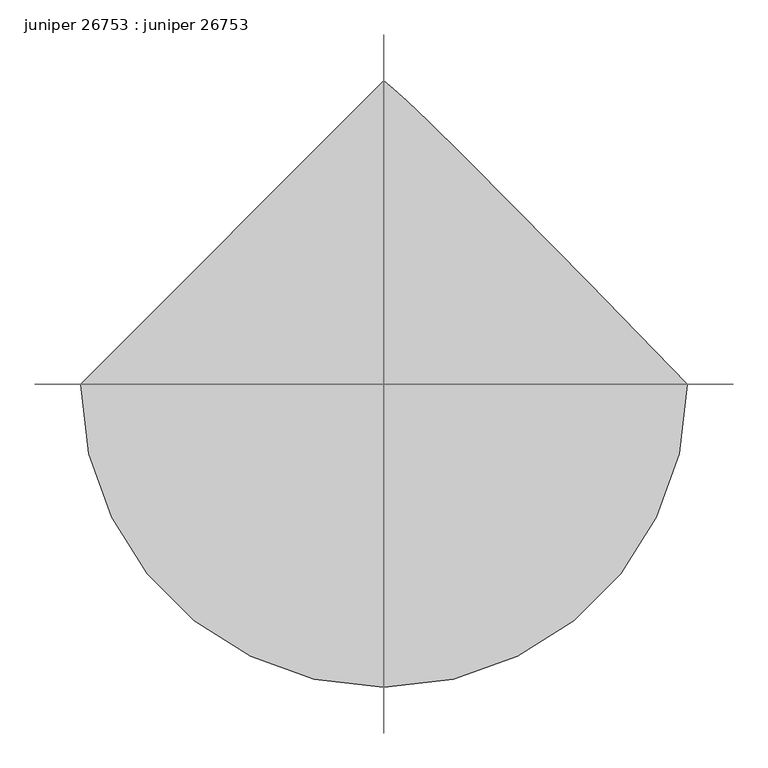
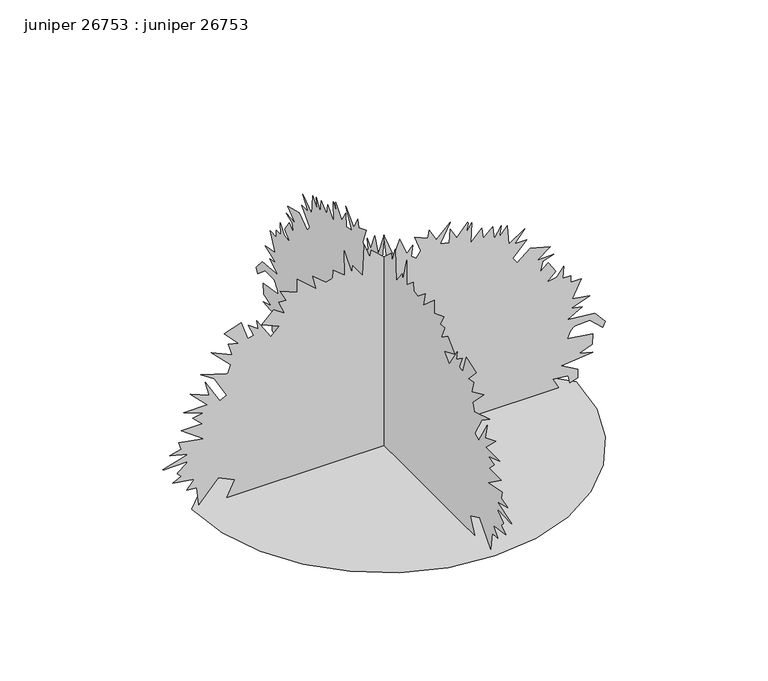
"""IFC4 building model written with IfcOpenShell, lengths in millimetres: proxy geometry, juniper 26753 : juniper 26753."""

from ifc_helpers import new_model, si_unit, origin, place, context, project, spatial, triangles, source, transform, mapped, element, save


def juniper_26753_juniper_26753_31b723d7(model_context):
    return source(origin(), model_context, "Body", "Tessellation", [
        triangles([(-789.9406637, 0.0, 7.34e-05), (-769.0593075, -181.0023239, 7.34e-05), (-709.58256, -347.2233553, 7.34e-05), (-616.27561, -493.9033919, 7.34e-05), (-493.9033919, -616.27561, 7.34e-05), (-347.2233553, -709.58256, 7.34e-05), (-181.0023239, -769.0593075, 7.34e-05), (3.45e-05, -789.9406637, 7.34e-05), (181.0025783, -769.0593075, 7.34e-05), (347.2233553, -709.58256, 7.34e-05), (493.9033919, -616.27561, 7.34e-05), (616.27561, -493.9033919, 7.34e-05), (709.58256, -347.2233553, 7.34e-05), (769.0593075, -181.0023239, 7.34e-05), (789.9406637, 6.91e-05, 7.34e-05), (533.2276995, 263.324552, 7.34e-05), (342.9129716, 457.2003633, 7.34e-05), (207.9314215, 593.1996929, 7.34e-05), (117.2157559, 682.8973429, 7.34e-05), (59.6994447, 737.8705862, 7.34e-05), (24.316455, 769.6942978, 7.34e-05), (-0.0001036, 789.9406637, 7.34e-05), (-3.6e-06, -645.975832, 2.9e-06), (1e-06, -614.2334381, 66.8205943), (0.0, -680.8932501, 98.5983058), (0.0, -760.2505428, 9.7171587), (0.0, -769.7755428, 85.9010885), (0.0, -811.0403933, 89.0753315), (0.0, -779.2979994, 127.1672379), (0.0, -868.1777487, 139.8647005), (0.0, -833.2603306, 158.9106491), (0.0, -849.1328356, 174.7823729), (2e-07, -847.0271502, 178.352086), (-1e-07, -810.1082554, 207.9471727), (0.0, -807.8654417, 212.8742702), (2e-07, -903.2958086, 210.5745559), (0.0, -909.4452152, 212.8742702), (0.0, -804.6929609, 244.6174271), (0.0, -880.8752295, 263.6623765), (0.0, -833.2603306, 276.3598392), (0.0, -842.7828598, 308.1047765), (0.0, -741.2056297, 289.0573199), (0.0, -833.2603306, 355.7196754), (0.0, -747.5530621, 355.7196754), (0.0, -785.6455044, 393.8120813), (0.0, -741.2056297, 403.3345379), (0.0, -823.737874, 431.9019439), (0.0, -725.3331247, 431.9019439), (0.0, -795.1679609, 501.7392872), (0.0, -718.9856924, 469.9943499), (0.0, -734.8581247, 533.4817174), (0.0, -674.5432743, 431.9019439), (0.0, -645.975832, 444.5994246), (0.0, -696.7657551, 533.4817174), (0.0, -753.9031105, 571.5741234), (0.0, -642.8008804, 536.6567053), (0.0, -630.1033997, 571.5741234), (0.0, -709.4632359, 650.9314161), (0.0, -623.7558947, 612.8389738), (0.0, -639.6283997, 663.6288969), (0.0, -598.3609694, 654.1063677), (0.0, -655.4982885, 714.4187473), (0.0, -585.663525, 739.8137089), (0.0, -560.2685635, 660.4538727), (0.0, -534.8736382, 666.8038485), (0.0, -557.0935756, 717.5912281), (0.0, -515.8286888, 689.0237858), (6e-07, -522.1761575, 724.2739597), (0.0, -465.0388021, 635.0589111), (0.0, -430.1214203, 669.9763292), (0.0, -503.131208, 701.7212666), (0.0, -452.3413576, 749.3361654), (0.0, -407.901483, 717.5912281), (0.0, -433.2964082, 774.731127), (0.0, -401.5514709, 771.5561028), (0.0, -426.9463961, 819.1710016), (0.0, -357.1115962, 790.6010159), (0.0, -357.1115962, 847.7409147), (0.0, -277.7543035, 777.9035351), (0.0, -293.6242287, 838.2159147), (0.0, -239.6616431, 793.7760401), (0.0, -211.0929654, 800.1260159), (0.0, -207.9182137, 835.043434), (0.0, -160.303333, 796.9510643), (0.0, -163.4780847, 904.8782701), (0.0, -131.7346644, 796.9510643), (0.0, -128.560167, 825.518434), (0.0, -87.2937723, 768.3810785), (0.0, -80.9452954, 901.7032459), (0.0, -58.7248448, 838.2159147), (0.0, -52.3763679, 866.7858278), (0.0, 11.1100709, 809.6484724), (0.0, -1.5869882, 914.4007267), (0.0, 39.6794049, 809.6484724), (0.0, 65.073835, 873.1333328), (0.0, 93.6427671, 800.1260159), (0.0, 119.037447, 828.6934582), (0.0, 112.6887157, 784.2535835), (0.0, 131.7349187, 768.3810785), (0.0, 150.7808674, 793.7760401), (0.0, 125.3861874, 860.4383955), (0.0, 179.3497903, 838.2159147), (0.0, 185.698022, 869.9608521), (0.0, 214.2674628, 819.1710016), (0.0, 271.4042913, 876.308357), (0.0, 230.1389141, 796.9510643), (0.0, 268.2318287, 787.4285351), (0.0, 271.4042913, 844.5658905), (0.0, 299.9742408, 796.9510643), (0.0, 342.3973417, 848.8686802), (0.0, 344.7290671, 848.6756687), (0.0, 345.397086, 844.7309967), (0.0, 338.0666468, 806.4735209), (0.0, 360.2865841, 841.3909389), (0.0, 357.1115962, 755.6835978), (0.0, 401.5540143, 803.2984966), (0.0, 407.901483, 758.858622), (0.0, 445.993889, 793.7760401), (0.0, 452.3413576, 739.8137089), (0.0, 480.9112707, 787.4285351), (0.0, 474.5612949, 739.8137089), (0.0, 506.3062323, 777.9035351), (0.0, 512.6537009, 695.3712908), (0.0, 579.3160563, 739.8137089), (0.0, 538.0486261, 689.0237858), (0.0, 585.663525, 689.0237858), (0.0, 528.5261696, 628.7114788), (0.0, 547.5710827, 603.3165173), (0.0, 601.5359937, 647.7563919), (0.0, 684.0682743, 625.5364546), (0.0, 630.1033997, 584.2716042), (0.0, 696.7657551, 587.4440486), (0.0, 652.3258804, 571.5741234), (0.0, 642.8008804, 530.3066932), (0.0, 674.5458178, 558.8766426), (0.0, 706.2882116, 511.2617801), (0.0, 668.1957693, 476.344362), (0.0, 709.4632359, 482.6918306), (0.0, 738.0306055, 520.7842366), (0.0, 734.8581247, 469.9943499), (0.0, 766.6005186, 469.9943499), (0.0, 766.6005186, 441.4269439), (0.0, 811.0403933, 441.4269439), (0.0, 772.9480236, 368.4171198), (0.0, 845.9578114, 355.7196754), (0.0, 769.7755428, 327.1497259), (0.0, 814.2154175, 317.6272694), (0.0, 753.9031105, 282.7098513), (0.0, 865.0053406, 273.1873765), (0.0, 909.4452152, 222.3972354), (0.0, 899.922686, 200.1767894), (0.0, 845.9578114, 247.7916701), (0.0, 785.3051182, 246.4035645), (0.0, 777.2710882, 242.5165924), (0.0, 770.76618, 236.5473347), (0.0, 765.4803835, 228.9123538), (0.0, 761.1116095, 220.0279215), (0.0, 757.3549347, 210.3106367), (0.0, 753.9031105, 200.1767894), (0.0, 858.6552921, 184.3053381), (0.0, 855.4828114, 139.8647005), (0.0, 801.5179367, 120.8187518), (0.0, 858.6552921, 104.9470462), (0.0, 728.508149, 92.2498288), (0.0, 795.1705044, 54.1576681), (0.0, 795.1705044, 16.0658174), (0.0, 763.4255671, 6.5428419), (0.0, 757.0780621, 38.2862123), (0.0, 693.5907309, 44.6346938), (0.0, 718.9856924, 0.1941814), (-645.975832, 0.000119, 0.0), (-614.2334381, 0.0001104, 66.8205943), (-680.8932501, 0.0001095, 98.5983058), (-760.2505428, 0.0001148, 9.7171587), (-769.7755428, 0.0001102, 85.9010885), (-811.0403933, 0.0001101, 89.0753315), (-779.2979994, 0.0001078, 127.1672379), (-868.1777487, 0.000107, 139.8647005), (-833.2603306, 0.0001059, 158.9106491), (-849.1328356, 0.0001049, 174.7823729), (-847.0271502, 0.0001045, 178.352086), (-810.1082554, 0.000103, 207.9471727), (-807.8654417, 0.0001027, 212.8742702), (-903.2958086, 0.0001026, 210.5745559), (-909.4452152, 0.0001027, 212.8742702), (-804.6929609, 0.0001008, 244.6174271), (-880.8752295, 9.97e-05, 263.6623765), (-833.2603306, 9.89e-05, 276.3598392), (-842.7828598, 9.7e-05, 308.1047765), (-741.2056297, 9.81e-05, 289.0573199), (-833.2603306, 9.42e-05, 355.7196754), (-747.5530621, 9.42e-05, 355.7196754), (-785.6455044, 9.19e-05, 393.8120813), (-741.2056297, 9.13e-05, 403.3345379), (-823.737874, 8.96e-05, 431.9019439), (-725.3331247, 8.96e-05, 431.9019439), (-795.1679609, 8.55e-05, 501.7367437), (-718.9856924, 8.74e-05, 469.9943499), (-734.8581247, 8.36e-05, 533.4817174), (-674.5458178, 8.96e-05, 431.9019439), (-645.975832, 8.89e-05, 444.5994246), (-696.7657551, 8.36e-05, 533.4817174), (-753.9031105, 8.13e-05, 571.5741234), (-642.8008804, 8.34e-05, 536.6567053), (-630.1033997, 8.13e-05, 571.5741234), (-709.4632359, 7.66e-05, 650.9314161), (-623.7558947, 7.88e-05, 612.8389738), (-639.6283997, 7.58e-05, 663.6288969), (-598.3609694, 7.64e-05, 654.1063677), (-655.4982885, 7.28e-05, 714.4187473), (-585.663525, 7.13e-05, 739.8137089), (-560.2685635, 7.6e-05, 660.4538727), (-534.8736382, 7.56e-05, 666.8038485), (-557.0935756, 7.26e-05, 717.5912281), (-515.8286888, 7.43e-05, 689.0237858), (-522.1761575, 7.16e-05, 724.2739597), (-465.0388021, 7.75e-05, 635.0589111), (-430.1214203, 7.54e-05, 669.9763292), (-503.131208, 7.35e-05, 701.7212666), (-452.3413576, 7.07e-05, 749.3361654), (-407.901483, 7.26e-05, 717.5912281), (-433.2964082, 6.92e-05, 774.731127), (-401.5540143, 6.94e-05, 771.5561028), (-426.9463961, 6.65e-05, 819.1710016), (-357.1115962, 6.82e-05, 790.6010159), (-357.1115962, 6.48e-05, 847.7409147), (-277.7543035, 6.9e-05, 777.9035351), (-293.6242287, 6.54e-05, 838.2159147), (-239.6616431, 6.81e-05, 793.7760401), (-211.0929654, 6.77e-05, 800.1260159), (-207.918468, 6.56e-05, 835.043434), (-160.303333, 6.79e-05, 796.9510643), (-163.4780847, 6.14e-05, 904.8782701), (-131.7349187, 6.79e-05, 796.9510643), (-128.560167, 6.62e-05, 825.518434), (-87.2940267, 6.96e-05, 768.3810785), (-80.9452954, 6.16e-05, 901.7032459), (-58.7250992, 6.54e-05, 838.2159147), (-52.3766177, 6.37e-05, 866.7858278), (11.1099687, 6.71e-05, 809.6484724), (-1.5870796, 6.09e-05, 914.4007267), (39.6791505, 6.71e-05, 809.6484724), (65.073835, 6.33e-05, 873.1333328), (93.6427671, 6.77e-05, 800.1260159), (119.037447, 6.6e-05, 828.6934582), (112.6887157, 6.86e-05, 784.2535835), (131.7346644, 6.96e-05, 768.3810785), (150.780613, 6.81e-05, 793.7760401), (125.3861874, 6.41e-05, 860.4358521), (179.349536, 6.54e-05, 838.2159147), (185.698022, 6.35e-05, 869.9608521), (214.2672084, 6.65e-05, 819.1710016), (271.4042913, 6.31e-05, 876.308357), (230.1389141, 6.79e-05, 796.9510643), (268.2318287, 6.84e-05, 787.4285351), (271.4042913, 6.5e-05, 844.5658905), (299.9742408, 6.79e-05, 796.9510643), (342.3973417, 6.48e-05, 848.8686802), (344.7290671, 6.48e-05, 848.6756687), (345.3945425, 6.5e-05, 844.7309967), (338.0666468, 6.73e-05, 806.4735209), (360.2865841, 6.52e-05, 841.3909389), (357.1115962, 7.03e-05, 755.6835978), (401.5514709, 6.75e-05, 803.2984966), (407.901483, 7.01e-05, 758.858622), (445.993889, 6.81e-05, 793.7760401), (452.3413576, 7.13e-05, 739.8137089), (480.9112707, 6.84e-05, 787.4285351), (474.5612949, 7.13e-05, 739.8137089), (506.3062323, 6.9e-05, 777.9035351), (512.6537009, 7.39e-05, 695.3712908), (579.3160563, 7.13e-05, 739.8137089), (538.0486261, 7.43e-05, 689.0237858), (585.663525, 7.43e-05, 689.0237858), (528.5261696, 7.79e-05, 628.7114788), (547.5710827, 7.94e-05, 603.3165173), (601.5359937, 7.68e-05, 647.7563919), (684.0682743, 7.81e-05, 625.5364546), (630.1033997, 8.05e-05, 584.2716042), (696.7657551, 8.04e-05, 587.4440486), (652.3258804, 8.13e-05, 571.5741234), (642.8008804, 8.38e-05, 530.3066932), (674.5458178, 8.21e-05, 558.8766426), (706.2882116, 8.49e-05, 511.2617801), (668.1957693, 8.7e-05, 476.344362), (709.4632359, 8.66e-05, 482.6918306), (738.0306055, 8.43e-05, 520.7842366), (734.8581247, 8.74e-05, 469.9943499), (766.6005186, 8.74e-05, 469.9943499), (766.6005186, 8.91e-05, 441.4269439), (811.0403933, 8.91e-05, 441.4269439), (772.9480236, 9.34e-05, 368.4171198), (845.9578114, 9.42e-05, 355.7196754), (769.7755428, 9.59e-05, 327.1497259), (814.2154175, 9.64e-05, 317.6272694), (753.9031105, 9.85e-05, 282.7098513), (865.0053406, 9.91e-05, 273.1873765), (909.4452152, 0.0001021, 222.3972354), (899.922686, 0.0001034, 200.1767894), (845.9578114, 0.0001006, 247.7916701), (785.3051182, 0.0001007, 246.4035645), (777.2710882, 0.0001009, 242.5165924), (770.76618, 0.0001013, 236.5473347), (765.4803835, 0.0001017, 228.9123538), (761.1116095, 0.0001023, 220.0279215), (757.3549347, 0.0001028, 210.3106367), (753.9031105, 0.0001034, 200.1767894), (858.6552921, 0.0001044, 184.3050838), (855.4828114, 0.000107, 139.8647005), (801.5179367, 0.0001082, 120.8187518), (858.6552921, 0.0001091, 104.9470462), (728.508149, 0.0001099, 92.2495745), (795.1705044, 0.0001121, 54.1576681), (795.1705044, 0.0001144, 16.0658174), (763.4255671, 0.000115, 6.5428419), (757.0780621, 0.0001131, 38.2862123), (693.5907309, 0.0001127, 44.6346938), (718.9856924, 0.0001154, 0.1941786)], [[21, 22, 1], [20, 21, 1], [19, 20, 1], [18, 19, 1], [17, 18, 1], [17, 1, 2], [17, 2, 3], [17, 3, 4], [16, 17, 4], [16, 4, 5], [16, 5, 6], [16, 6, 7], [16, 7, 8], [16, 8, 9], [16, 9, 10], [16, 10, 11], [16, 11, 12], [15, 16, 12], [14, 15, 12], [13, 14, 12], [92, 93, 94], [84, 85, 86], [54, 55, 56], [50, 51, 52], [131, 132, 133], [123, 124, 125], [104, 105, 106], [46, 47, 48], [57, 58, 59], [88, 89, 90], [48, 49, 50], [67, 68, 69], [119, 120, 121], [162, 163, 164], [38, 39, 40], [113, 114, 115], [144, 145, 146], [65, 66, 67], [138, 139, 140], [96, 97, 98], [107, 108, 109], [79, 80, 81], [42, 43, 44], [29, 30, 31], [36, 37, 38], [75, 76, 77], [102, 103, 104], [146, 147, 148], [86, 87, 88], [94, 95, 96], [121, 122, 123], [125, 126, 127], [100, 101, 102], [77, 78, 79], [25, 26, 27], [115, 116, 117], [129, 130, 131], [117, 118, 119], [27, 28, 29], [82, 83, 84], [44, 45, 46], [48, 50, 52], [59, 60, 61], [169, 170, 23], [73, 74, 75], [90, 91, 92], [142, 143, 144], [40, 41, 42], [38, 40, 42], [169, 23, 24], [53, 54, 56], [61, 62, 63], [61, 63, 64], [70, 71, 72], [70, 72, 73], [150, 151, 152], [149, 150, 152], [148, 149, 152], [148, 152, 153], [128, 129, 131], [148, 153, 154], [35, 36, 38], [134, 135, 136], [134, 136, 137], [65, 67, 69], [166, 167, 168], [165, 166, 168], [164, 165, 168], [164, 168, 169], [88, 90, 92], [140, 141, 142], [100, 102, 104], [159, 160, 161], [159, 161, 162], [25, 27, 29], [123, 125, 127], [148, 154, 155], [100, 104, 106], [110, 111, 112], [109, 110, 112], [109, 112, 113], [109, 113, 115], [31, 32, 33], [131, 133, 134], [159, 162, 164], [128, 131, 134], [46, 48, 52], [73, 75, 77], [73, 77, 79], [29, 31, 33], [29, 33, 34], [44, 46, 52], [148, 155, 156], [164, 169, 24], [159, 164, 24], [158, 159, 24], [157, 158, 24], [156, 157, 24], [148, 156, 24], [146, 148, 24], [144, 146, 24], [142, 144, 24], [140, 142, 24], [138, 140, 24], [137, 138, 24], [134, 137, 24], [128, 134, 24], [127, 128, 24], [123, 127, 24], [121, 123, 24], [119, 121, 24], [117, 119, 24], [115, 117, 24], [109, 115, 24], [107, 109, 24], [106, 107, 24], [106, 24, 25], [106, 25, 29], [106, 29, 34], [106, 34, 35], [106, 35, 38], [106, 38, 42], [106, 42, 44], [106, 44, 52], [106, 52, 53], [106, 53, 56], [99, 100, 106], [99, 106, 56], [99, 56, 57], [98, 99, 57], [96, 98, 57], [94, 96, 57], [59, 61, 64], [57, 59, 64], [70, 73, 79], [64, 65, 69], [57, 64, 69], [94, 57, 69], [84, 86, 88], [88, 92, 94], [88, 94, 69], [88, 69, 70], [88, 70, 79], [84, 88, 79], [82, 84, 79], [82, 79, 81], [240, 241, 242], [232, 233, 234], [202, 203, 204], [198, 199, 200], [279, 280, 281], [271, 272, 273], [252, 253, 254], [194, 195, 196], [205, 206, 207], [236, 237, 238], [196, 197, 198], [215, 216, 217], [267, 268, 269], [310, 311, 312], [186, 187, 188], [261, 262, 263], [292, 293, 294], [213, 214, 215], [286, 287, 288], [244, 245, 246], [255, 256, 257], [227, 228, 229], [190, 191, 192], [177, 178, 179], [184, 185, 186], [223, 224, 225], [250, 251, 252], [294, 295, 296], [234, 235, 236], [242, 243, 244], [269, 270, 271], [273, 274, 275], [248, 249, 250], [225, 226, 227], [173, 174, 175], [263, 264, 265], [277, 278, 279], [265, 266, 267], [175, 176, 177], [230, 231, 232], [192, 193, 194], [196, 198, 200], [207, 208, 209], [317, 318, 171], [221, 222, 223], [238, 239, 240], [290, 291, 292], [188, 189, 190], [186, 188, 190], [317, 171, 172], [201, 202, 204], [209, 210, 211], [209, 211, 212], [218, 219, 220], [218, 220, 221], [298, 299, 300], [297, 298, 300], [296, 297, 300], [296, 300, 301], [276, 277, 279], [296, 301, 302], [183, 184, 186], [282, 283, 284], [282, 284, 285], [213, 215, 217], [314, 315, 316], [313, 314, 316], [312, 313, 316], [312, 316, 317], [236, 238, 240], [288, 289, 290], [248, 250, 252], [307, 308, 309], [307, 309, 310], [173, 175, 177], [271, 273, 275], [296, 302, 303], [248, 252, 254], [258, 259, 260], [257, 258, 260], [257, 260, 261], [257, 261, 263], [179, 180, 181], [279, 281, 282], [307, 310, 312], [276, 279, 282], [194, 196, 200], [221, 223, 225], [221, 225, 227], [177, 179, 181], [177, 181, 182], [192, 194, 200], [296, 303, 304], [312, 317, 172], [307, 312, 172], [306, 307, 172], [305, 306, 172], [304, 305, 172], [296, 304, 172], [294, 296, 172], [292, 294, 172], [290, 292, 172], [288, 290, 172], [286, 288, 172], [285, 286, 172], [282, 285, 172], [276, 282, 172], [275, 276, 172], [271, 275, 172], [269, 271, 172], [267, 269, 172], [265, 267, 172], [263, 265, 172], [257, 263, 172], [255, 257, 172], [254, 255, 172], [254, 172, 173], [254, 173, 177], [254, 177, 182], [254, 182, 183], [254, 183, 186], [254, 186, 190], [254, 190, 192], [254, 192, 200], [254, 200, 201], [254, 201, 204], [247, 248, 254], [247, 254, 204], [247, 204, 205], [246, 247, 205], [244, 246, 205], [242, 244, 205], [207, 209, 212], [205, 207, 212], [218, 221, 227], [212, 213, 217], [205, 212, 217], [242, 205, 217], [232, 234, 236], [236, 240, 242], [236, 242, 217], [236, 217, 218], [236, 218, 227], [232, 236, 227], [230, 232, 227], [230, 227, 229]], closed=False),
    ])


if __name__ == "__main__":
    model = new_model("IFC4")
    model_context = context("Model", 3, world=origin())
    ifc_project = project(units=[si_unit("LENGTHUNIT", "METRE", prefix="MILLI")], contexts=[model_context])
    site = spatial("IfcSite", under=ifc_project)
    building = spatial("IfcBuilding", under=site)
    placement = place(None, origin())
    juniper_26753_juniper_26753_shape = juniper_26753_juniper_26753_31b723d7(model_context)
    element("IfcBuildingElementProxy", 1, Name="juniper 26753 : juniper 26753", ObjectType="juniper 26753 : juniper 26753", at=placement, inside=building, context=model_context, shape_type="MappedRepresentation", body=[
        mapped(juniper_26753_juniper_26753_shape, transform((0.0, 0.0, 0.0), x_axis=(1.0, 0.0, 0.0), y_axis=(0.0, 1.0, 0.0), z_axis=(0.0, 0.0, 1.0))),
    ])
    save(model, "model.ifc")

# Revit data of these elements
# Type "juniper 26753 : juniper 26753"
#   built-in parameter 1005195 = "RPC-16-FU4H-UTPX-8HVP-A000-ST1L-LVER-AU"
#   Height = 0
